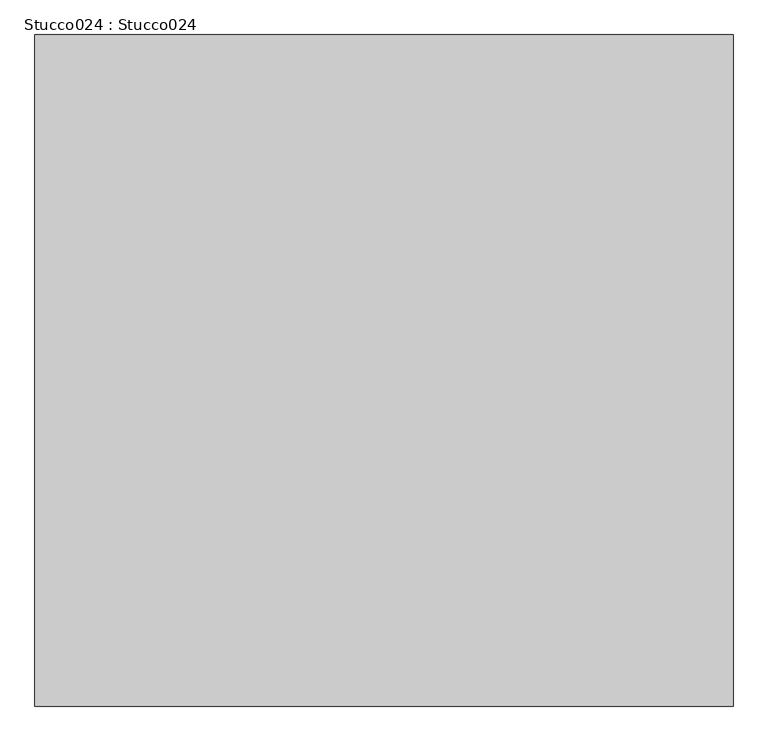
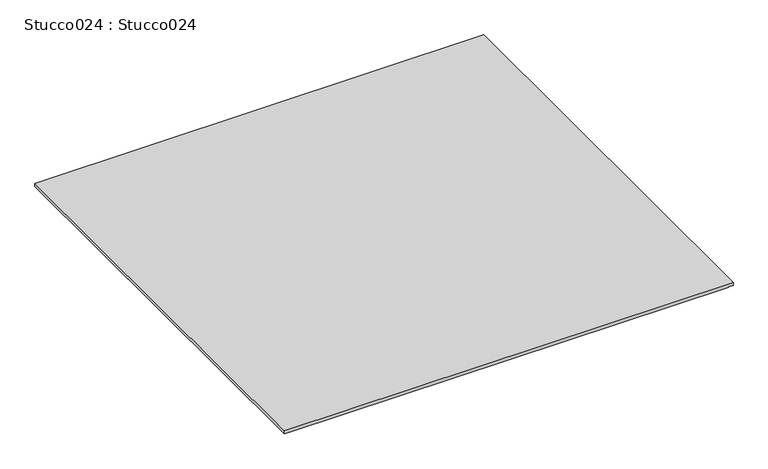
"""IFC4 building model written with IfcOpenShell, lengths in millimetres: proxy geometry, Stucco024 : Stucco024."""

from ifc_helpers import new_model, si_unit, frame, origin, place, context, project, spatial, polyline, outline, extrude, source, transform, mapped, element, save


def stucco024_stucco024_65a95bb4(model_context):
    return source(origin(), model_context, "Body", "SweptSolid", [
        extrude(outline(polyline([(39545.1675708, -2732.0873925), (39543.8875708, -2732.0873925), (39543.8875708, -697.84966), (39545.1675708, -697.84966), (39545.1675708, -675.416476), (39560.2460083, -675.416476), (39560.2460083, -2754.5205764), (39545.1675708, -2754.5205764), (39545.1675708, -2732.0873925)])), frame((0.0, -1052.8906574, 0.0), z_axis=(0.0, 1.0, 0.0), x_axis=(0.0, 0.0, 1.0)), (0.0, 0.0, 1.0), 2000.0),
    ])


if __name__ == "__main__":
    model = new_model("IFC4")
    model_context = context("Model", 3, world=origin())
    ifc_project = project(units=[si_unit("LENGTHUNIT", "METRE", prefix="MILLI")], contexts=[model_context])
    site = spatial("IfcSite", under=ifc_project)
    building = spatial("IfcBuilding", under=site)
    placement = place(None, origin())
    stucco024_stucco024_shape = stucco024_stucco024_65a95bb4(model_context)
    element("IfcBuildingElementProxy", 1, Name="Stucco024 : Stucco024", ObjectType="Stucco024 : Stucco024", at=placement, inside=building, context=model_context, shape_type="MappedRepresentation", body=[
        mapped(stucco024_stucco024_shape, transform((0.0, 0.0, 0.0), x_axis=(1.0, 0.0, 0.0), y_axis=(0.0, 1.0, 0.0), z_axis=(0.0, 0.0, 1.0))),
    ])
    save(model, "model.ifc")

# Revit data of these elements
# Type "Stucco024 : Stucco024"
#   NameOverride = "Stucco024"
# Element 1 (IfcBuildingElementProxy, "Stucco024 : Stucco024")
#   Materials on its faces: "7/8\" SMOOTH TROWEL EXTERIOR STUCCO"
# Materials
#   "7/8\" SMOOTH TROWEL EXTERIOR STUCCO": class "Unassigned", colour RGB 255 255 255, transparency 0, Cost = 0
